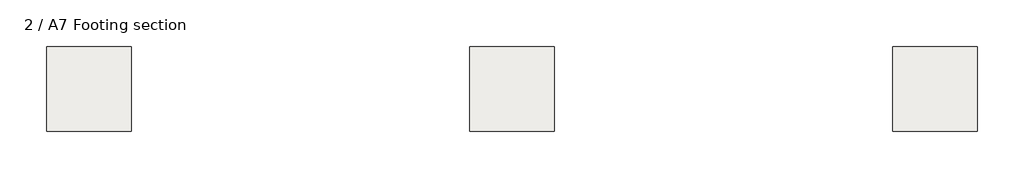
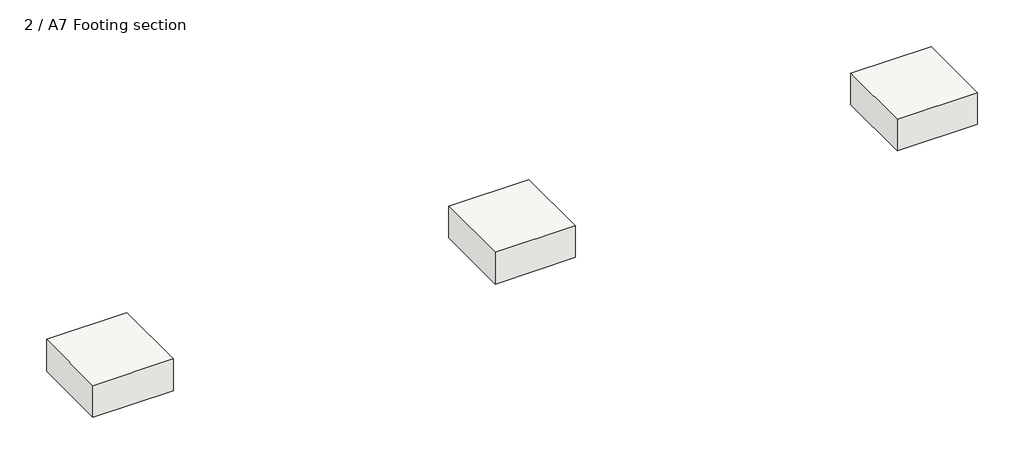
# One storey, part 1 of 2: 3 slabs.
"""IFC4 building model written with IfcOpenShell, lengths in millimetres."""

import ifcopenshell
import ifcopenshell.guid

model = None  # the IFC model being written
_history = None  # IfcOwnerHistory: only IFC2X3 demands one
_inside = {}  # id of a spatial element -> (the spatial element, [elements in it])
_under = {}  # id of a project, library or spatial element -> (it, [spatial elements below it])
_declared = {}  # id of a project -> (the project, [libraries it declares])
_typed = {}  # id of a type object -> (the type object, [elements of that type])
_made_of = {}  # id of a material, layer set ... -> (it, [elements and type objects made of it])


def new_model(schema):
    """Start an empty IFC model of exactly this schema.

    Asked for "IFC4X3", IfcOpenShell would pick the latest addendum, in which some entities
    have other attributes; the version numbers below select the first issue.
    IFC2X3 requires an IfcOwnerHistory on every rooted entity: one is made here for all.
    """
    global model, _history
    if schema == "IFC4X3":
        model = ifcopenshell.file(schema_version=(4, 3, 0, 0))
    else:
        model = ifcopenshell.file(schema=schema)
    _inside.clear()
    _under.clear()
    _declared.clear()
    _typed.clear()
    _made_of.clear()
    _history = None
    if model.schema == "IFC2X3":
        org = make("IfcOrganization", Name="unknown")
        user = make(
            "IfcPersonAndOrganization",
            ThePerson=make("IfcPerson", FamilyName="unknown"),
            TheOrganization=org,
        )
        app = make(
            "IfcApplication",
            ApplicationDeveloper=org,
            Version="unknown",
            ApplicationFullName="unknown",
            ApplicationIdentifier="unknown",
        )
        _history = make(
            "IfcOwnerHistory",
            OwningUser=user,
            OwningApplication=app,
            ChangeAction="ADDED",
            CreationDate=0,
        )
    return model


def make(cls, **values):
    """One entity of the class cls with the attributes given. An attribute that is None is left unset."""
    return model.create_entity(
        cls, **{name: value for name, value in values.items() if value is not None}
    )


def rooted(cls, **values):
    """An entity with a GlobalId (a new one), such as an element, a storey or a relation."""
    return make(cls, GlobalId=ifcopenshell.guid.new(), OwnerHistory=_history, **values)


def si_unit(unit_type, name, prefix=None):
    """IfcSIUnit, for example si_unit("LENGTHUNIT", "METRE", prefix="MILLI")."""
    return make("IfcSIUnit", UnitType=unit_type, Prefix=prefix, Name=name)


def assignment(units):
    """IfcUnitAssignment: the units of a project."""
    return None if units is None else make("IfcUnitAssignment", Units=units)


def point(xyz):
    """IfcCartesianPoint."""
    return None if xyz is None else make("IfcCartesianPoint", Coordinates=xyz)


def direction(xyz):
    """IfcDirection."""
    return None if xyz is None else make("IfcDirection", DirectionRatios=xyz)


def frame(location, z_axis=None, x_axis=None):
    """IfcAxis2Placement3D, a coordinate frame: its origin and axes. An axis left out is left unset."""
    return make(
        "IfcAxis2Placement3D",
        Location=point(location),
        Axis=direction(z_axis),
        RefDirection=direction(x_axis),
    )


def origin():
    """The frame at (0, 0, 0) with its axes left unset."""
    return frame((0.0, 0.0, 0.0))


def place(relative_to, where):
    """IfcLocalPlacement: puts the frame where relative to a parent placement (None: the world)."""
    return make(
        "IfcLocalPlacement", PlacementRelTo=relative_to, RelativePlacement=where
    )


def context(
    kind, dimensions, precision=None, world=None, true_north=None, identifier=None
):
    """IfcGeometricRepresentationContext, for example the 3D "Model" context."""
    return make(
        "IfcGeometricRepresentationContext",
        ContextIdentifier=identifier,
        ContextType=kind,
        CoordinateSpaceDimension=dimensions,
        Precision=precision,
        WorldCoordinateSystem=world,
        TrueNorth=true_north,
    )


def project(units=None, contexts=None):
    """IfcProject with its units and contexts."""
    return rooted(
        "IfcProject",
        Name="project",
        RepresentationContexts=contexts,
        UnitsInContext=assignment(units),
    )


def spatial(cls, under=None, at=None, **own):
    """A site, building, storey or space (cls), placed at a placement, below another one or the project."""
    s = rooted(cls, ObjectPlacement=at, **own)
    if under is not None:
        _under.setdefault(under.id(), (under, []))[1].append(s)
    return s


def polyline(points):
    """IfcPolyline through the points."""
    return make("IfcPolyline", Points=[point(p) for p in points])


def outline(outer, holes=None, kind="AREA"):
    """IfcArbitraryClosedProfileDef: a profile drawn as a closed curve; with holes, ...WithVoids."""
    if holes is None:
        return make("IfcArbitraryClosedProfileDef", ProfileType=kind, OuterCurve=outer)
    return make(
        "IfcArbitraryProfileDefWithVoids",
        ProfileType=kind,
        OuterCurve=outer,
        InnerCurves=holes,
    )


def extrude(swept, where, along, depth):
    """IfcExtrudedAreaSolid: the profile swept, set in the frame where, extruded along a direction by depth."""
    return make(
        "IfcExtrudedAreaSolid",
        SweptArea=swept,
        Position=where,
        ExtrudedDirection=direction(along),
        Depth=depth,
    )


def shape(context_of_items, identifier, shape_type, items):
    """IfcShapeRepresentation: the items that make up one representation, for example the "Body"."""
    return make(
        "IfcShapeRepresentation",
        ContextOfItems=context_of_items,
        RepresentationIdentifier=identifier,
        RepresentationType=shape_type,
        Items=items,
    )


def source(mapping_origin, context_of_items, identifier, shape_type, items):
    """IfcRepresentationMap: a shape defined once, which mapped items show again and again."""
    return make(
        "IfcRepresentationMap",
        MappingOrigin=mapping_origin,
        MappedRepresentation=shape(context_of_items, identifier, shape_type, items),
    )


def transform(
    local_origin,
    x_axis=None,
    y_axis=None,
    z_axis=None,
    scale=None,
    scale2=None,
    scale3=None,
    uniform=True,
):
    """IfcCartesianTransformationOperator3D, or its non-uniform kind. x_axis, y_axis, z_axis: its Axis1, 2, 3."""
    if uniform:
        return make(
            "IfcCartesianTransformationOperator3D",
            Axis1=direction(x_axis),
            Axis2=direction(y_axis),
            LocalOrigin=point(local_origin),
            Scale=scale,
            Axis3=direction(z_axis),
        )
    return make(
        "IfcCartesianTransformationOperator3DnonUniform",
        Axis1=direction(x_axis),
        Axis2=direction(y_axis),
        LocalOrigin=point(local_origin),
        Scale=scale,
        Axis3=direction(z_axis),
        Scale2=scale2,
        Scale3=scale3,
    )


def mapped(mapping_source, mapping_target):
    """IfcMappedItem: shows the shape of a source again, moved by a transform."""
    return make(
        "IfcMappedItem", MappingSource=mapping_source, MappingTarget=mapping_target
    )


def made_of(thing, what):
    """Note that an element or type object is made of a material, layer set ...; save() writes the relation."""
    if what is not None:
        _made_of.setdefault(what.id(), (what, []))[1].append(thing)
    return thing


def element(
    cls,
    number,
    at=None,
    inside=None,
    cuts=None,
    type_object=None,
    material=None,
    context=None,
    identifier="Body",
    shape_type=None,
    held_by="IfcProductDefinitionShape",
    body=None,
    shapes=None,
    **own,
):
    """One element of the class cls, such as IfcWall. Its Tag is "e" and its number.

    at: its placement. inside: the storey or other place that contains it. cuts: it is an
    opening in that element (IfcRelVoidsElement). A single representation is given by context,
    identifier, shape_type and body (its items); several are given by shapes. held_by: the class
    of the entity that holds the representations. save() writes the other relations.
    """
    e = rooted(cls, Tag="e%d" % number, ObjectPlacement=at, **own)
    if body is not None:
        shapes = [shape(context, identifier, shape_type, body)]
    if shapes is not None:
        e.Representation = make(held_by, Representations=shapes)
    if inside is not None:
        _inside.setdefault(inside.id(), (inside, []))[1].append(e)
    if cuts is not None:
        rooted(
            "IfcRelVoidsElement", RelatingBuildingElement=cuts, RelatedOpeningElement=e
        )
    if type_object is not None:
        _typed.setdefault(type_object.id(), (type_object, []))[1].append(e)
    return made_of(e, material)


def aggregate(whole, parts):
    """IfcRelAggregates: a whole, such as a stair, and the parts it consists of."""
    return rooted("IfcRelAggregates", RelatingObject=whole, RelatedObjects=parts)


def save(model, path):
    """Write the relations noted so far, then the file.

    IfcRelAggregates (storeys below a building ...), IfcRelContainedInSpatialStructure (elements
    in a storey), IfcRelDefinesByType, IfcRelAssociatesMaterial and IfcRelDeclares: one each for
    every whole, place, type object, material and project.
    """
    for whole, parts in _under.values():
        aggregate(whole, parts)
    for where, things in _inside.values():
        rooted(
            "IfcRelContainedInSpatialStructure",
            RelatedElements=things,
            RelatingStructure=where,
        )
    for kind, things in _typed.values():
        rooted("IfcRelDefinesByType", RelatedObjects=things, RelatingType=kind)
    for what, things in _made_of.values():
        rooted("IfcRelAssociatesMaterial", RelatedObjects=things, RelatingMaterial=what)
    for by, libraries in _declared.values():
        rooted("IfcRelDeclares", RelatingContext=by, RelatedDefinitions=libraries)
    model.write(path)


def slab_7656c398(model_context):
    return source(origin(), model_context, "Body", "SweptSolid", [
        extrude(outline(polyline([(304.8, 304.8), (304.8, -304.8), (-304.8, -304.8), (-304.8, 304.8), (304.8, 304.8)])), frame((0.0, 0.0, -254.0), z_axis=(0.0, 0.0, 1.0), x_axis=(1.0, 0.0, 0.0)), (0.0, 0.0, 1.0), 254.0),
    ])


model = new_model("IFC4")

# Units and contexts
model_context = context("Model", 3, world=origin())
ifc_project = project(units=[si_unit("LENGTHUNIT", "METRE", prefix="MILLI")], contexts=[model_context])

# Site, building, storey
site = spatial("IfcSite", under=ifc_project)
building = spatial("IfcBuilding", under=site)
storey = spatial("IfcBuildingStorey", under=building, Name="2 / A7 Footing section", Elevation=-573.88125)

# Slabs
placement = place(None, origin())
slab_shape = slab_7656c398(model_context)
element("IfcSlab", 1, ObjectType="Footing-Rectangular : BLDG 6241 24\" x 24\" x 10\" Footing", at=placement, inside=storey, context=model_context, shape_type="MappedRepresentation", body=[
    mapped(slab_shape, transform((-1697.614829, 26.1284114, -573.88125), x_axis=(1.0, 0.0, 0.0), y_axis=(0.0, 1.0, 0.0), z_axis=(0.0, 0.0, 1.0))),
])
element("IfcSlab", 2, ObjectType="Footing-Rectangular : BLDG 6241 24\" x 24\" x 10\" Footing", at=placement, inside=storey, context=model_context, shape_type="MappedRepresentation", body=[
    mapped(slab_shape, transform((-4745.614829, 26.1284114, -573.88125), x_axis=(1.0, 0.0, 0.0), y_axis=(0.0, 1.0, 0.0), z_axis=(0.0, 0.0, 1.0))),
])
element("IfcSlab", 3, ObjectType="Footing-Rectangular : BLDG 6241 24\" x 24\" x 10\" Footing", at=placement, inside=storey, context=model_context, shape_type="MappedRepresentation", body=[
    mapped(slab_shape, transform((-7793.614829, 26.1284114, -573.88125), x_axis=(1.0, 0.0, 0.0), y_axis=(0.0, 1.0, 0.0), z_axis=(0.0, 0.0, 1.0))),
])

save(model, "model.ifc")

# Revit data of these elements
# Project information
#   Project Issue Date = "Issue Date"
#   Project Status = "Project Status"
#   Client Name = "Owner"
#   Project Address = "Enter address here"
#   Project Name = "Project Name"
#   Project Number = "Project Number"
# Grids (mm)
#   "X": line (-20839.361, 26.128) -> (5817.21, 26.128)
#   "1": line (-17801.215, 8272.214) -> (-17801.215, -7229.778)
#   "2": line (-11152.765, 8272.214) -> (-11152.765, -7229.778)
#   "3": line (-7438.015, 8272.214) -> (-7438.015, -7229.778)
#   "4": line (-6828.415, 8272.214) -> (-6828.415, -7229.778)
#   "5": line (-5609.215, 8272.214) -> (-5609.215, -7229.778)
#   "6": line (-2561.215, 8272.214) -> (-2561.215, -7229.778)
#   "7": line (-1951.615, 8272.214) -> (-1951.615, -7229.778)
#   "8": line (1705.985, 8272.214) -> (1705.985, -7229.778)
#   "A": line (-20839.361, 5207.728) -> (5817.21, 5207.728)
#   "B": line (-20839.361, 1226.278) -> (5817.21, 1226.278)
#   "C": line (-20839.361, -837.472) -> (5817.21, -837.472)
#   "D": line (-20839.361, -3529.872) -> (5817.21, -3529.872)
#   "E": line (-20839.361, -5053.872) -> (5817.21, -5053.872)
#   "G": line (-20839.361, -5155.472) -> (5817.21, -5155.472)
# Type "Footing-Rectangular : BLDG 6241 24\" x 24\" x 10\" Footing"
#   Assembly Code = "A1010100"
#   Width = 2' - 0"
#   Length = 2' - 0"
#   Foundation Thickness = 0' - 10"
#   Structural Material [instance default] = Concrete, Cast-in-Place gray
# Elements 1, 2, 3 (IfcSlab, "Footing-Rectangular : BLDG 6241 24\" x 24\" x 10\" Footing")
#   Comments = ""
#   Structural Material = BLDG 6241 Concrete(3500 psi)
#   Phase Created = New Construction
#   Materials on its faces: "BLDG 6241 Concrete(3500 psi)"
# Materials
#   "Concrete, Cast-in-Place gray": class "Concrete", colour RGB 192 192 192, transparency 0, Description = "Cast-in-place concrete", Cost = 0
#   "BLDG 6241 Concrete(3500 psi)": class "Concrete", colour RGB 127 127 127, transparency 0, Description = "Portland Cement Concrete", Cost = 0
